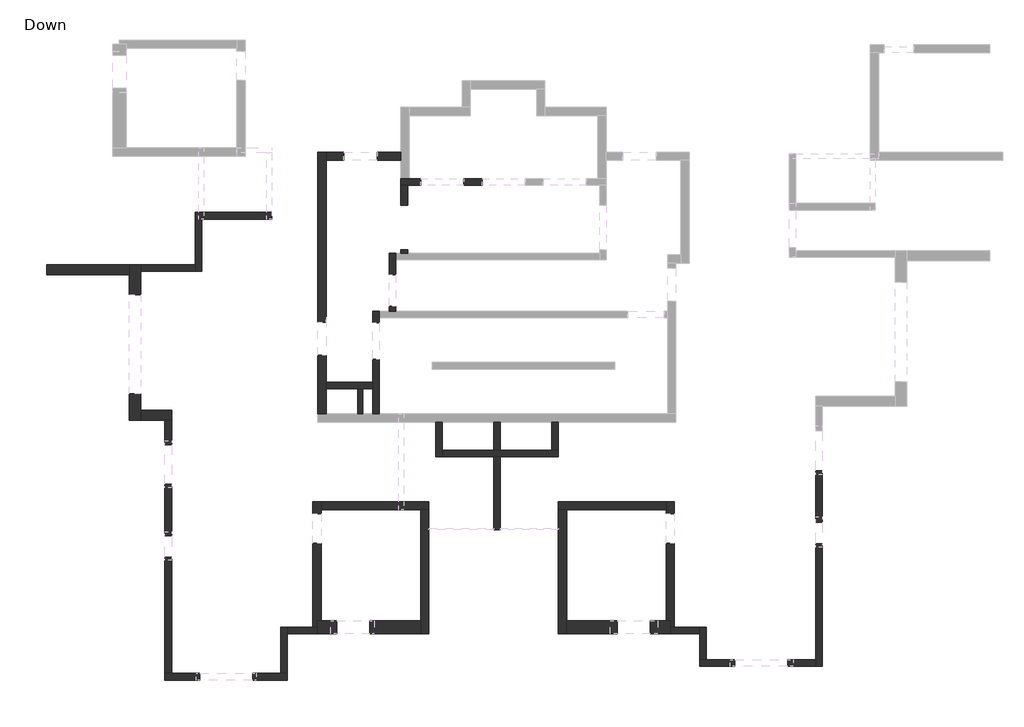
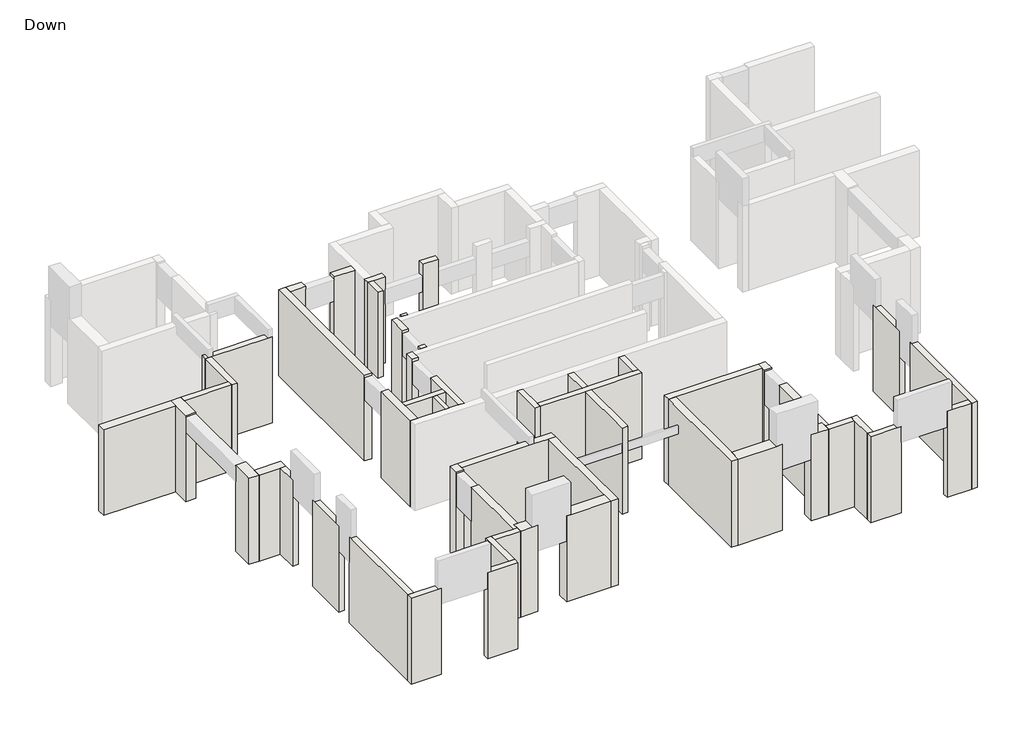
# One storey, part 1 of 3: 51 walls.
"""IFC4 building model written with IfcOpenShell, lengths in millimetres."""

from ifc_helpers import new_model, si_unit, origin, origin_with_axes, place, context, project, spatial, polyline, outline, extrude, faceted_brep, element, save

model = new_model("IFC4")

# Units and contexts
model_context = context("Model", 3, world=origin())
ifc_project = project(units=[si_unit("LENGTHUNIT", "METRE", prefix="MILLI")], contexts=[model_context])

# Site, building, storey
site = spatial("IfcSite", under=ifc_project)
building = spatial("IfcBuilding", under=site)
storey = spatial("IfcBuildingStorey", under=building, Name="Down", Elevation=0.0)

# Walls
placement = place(None, origin())
element("IfcWall", 1, ObjectType="15", at=placement, inside=storey, context=model_context, shape_type="SweptSolid", body=[
    extrude(outline(polyline([(-19501.573099, -7874.1201217), (-19501.573099, -7122.1728784), (-19351.573099, -7122.1728784), (-19351.573099, -7874.1201217), (-19501.573099, -7874.1201217)])), origin_with_axes(), (0.0, 0.0, 1.0), 3150.0),
])
element("IfcWall", 2, ObjectType="20", at=placement, inside=storey, context=model_context, shape_type="Brep", body=[
    faceted_brep([(-22100.9487358, -1784.190313, 0.0), (-24415.0622873, -1784.190313, 0.0), (-24415.0622873, -1784.190313, 3150.0), (-24310.0622873, -1784.190313, 3150.0), (-24160.0622873, -1784.190313, 3150.0), (-22250.9487358, -1784.190313, 3150.0), (-22100.9487358, -1784.190313, 3150.0), (-22100.9487358, -1784.190313, 2850.0), (-22100.9487358, -1984.190313, 0.0), (-22100.9487358, -1984.190313, 2950.0), (-22100.9487358, -1984.190313, 3150.0), (-22250.9487358, -1984.190313, 3150.0), (-24160.0622873, -1984.190313, 3150.0), (-24215.0622873, -1984.190313, 3150.0), (-24310.0622873, -1984.190313, 3150.0), (-24415.0622873, -1984.190313, 3150.0), (-24415.0622873, -1984.190313, 0.0), (-24215.0622873, -1984.190313, 0.0)], [[[0, 1, 2, 3, 4, 5, 6, 7]], [[8, 9, 10, 11, 12, 13, 14, 15, 16, 17]], [[1, 0, 8, 17, 16]], [[6, 5, 4, 3, 2, 15, 14, 13, 12, 11, 10]], [[0, 7, 6, 10, 9, 8]], [[2, 1, 16, 15]]]),
])
element("IfcWall", 3, ObjectType="20", at=placement, inside=storey, context=model_context, shape_type="Brep", body=[
    faceted_brep([(-24415.0622873, -1984.190313, 0.0), (-24415.0622873, -3366.82362, 0.0), (-24415.0622873, -3566.82362, 0.0), (-24415.0622873, -3566.82362, 3150.0), (-24415.0622873, -3366.82362, 3150.0), (-24415.0622873, -1984.190313, 3150.0), (-24215.0622873, -1984.190313, 0.0), (-24215.0622873, -1984.190313, 2950.0), (-24215.0622873, -1984.190313, 3150.0), (-24215.0622873, -3566.82362, 3150.0), (-24215.0622873, -3566.82362, 2950.0), (-24215.0622873, -3566.82362, 0.0)], [[[0, 1, 2, 3, 4, 5]], [[6, 7, 8, 9, 10, 11]], [[2, 1, 0, 6, 11]], [[5, 4, 3, 9, 8]], [[0, 5, 8, 7, 6]], [[3, 2, 11, 10, 9]]]),
])
element("IfcWall", 4, ObjectType="20", at=placement, inside=storey, context=model_context, shape_type="Brep", body=[
    faceted_brep([(-24415.0622873, -3366.82362, 0.0), (-26062.7923903, -3366.82362, 0.0), (-26062.7923903, -3366.82362, 3150.0), (-24415.0622873, -3366.82362, 3150.0), (-24415.0622873, -3566.82362, 0.0), (-24415.0622873, -3566.82362, 3150.0), (-26062.7923903, -3566.82362, 3150.0), (-26062.7923903, -3566.82362, 2950.0), (-26062.7923903, -3566.82362, 0.0)], [[[0, 1, 2, 3]], [[4, 5, 6, 7, 8]], [[1, 0, 4, 8]], [[3, 2, 6, 5]], [[0, 3, 5, 4]], [[2, 1, 8, 7, 6]]]),
])
element("IfcWall", 5, ObjectType="20", at=placement, inside=storey, context=model_context, shape_type="Brep", body=[
    faceted_brep([(-25331.1270445, -12221.0520814, 0.0), (-25331.1270445, -15727.4032645, 0.0), (-25331.1270445, -15727.4032645, 3150.0), (-25331.1270445, -12301.0520814, 3150.0), (-25331.1270445, -12221.0520814, 3150.0), (-25331.1270445, -12221.0520814, 2220.0), (-25131.1270445, -12221.0520814, 0.0), (-25131.1270445, -12221.0520814, 2220.0), (-25131.1270445, -12221.0520814, 3150.0), (-25131.1270445, -12301.0520814, 3150.0), (-25131.1270445, -15727.4032645, 3150.0), (-25131.1270445, -15727.4032645, 2950.0), (-25131.1270445, -15727.4032645, 0.0)], [[[0, 1, 2, 3, 4, 5]], [[6, 7, 8, 9, 10, 11, 12]], [[1, 0, 6, 12]], [[4, 3, 2, 10, 9, 8]], [[0, 5, 4, 8, 7, 6]], [[2, 1, 12, 11, 10]]]),
])
element("IfcWall", 6, ObjectType="20", at=placement, inside=storey, context=model_context, shape_type="Brep", body=[
    faceted_brep([(-22676.7174441, -15927.4032645, 0.0), (-21625.2739934, -15927.4032645, 0.0), (-21625.2739934, -15927.4032645, 3150.0), (-22565.2739934, -15927.4032645, 3150.0), (-22676.7174441, -15927.4032645, 3150.0), (-22676.7174441, -15927.4032645, 2570.0), (-22676.7174441, -15727.4032645, 0.0), (-22676.7174441, -15727.4032645, 2570.0), (-22676.7174441, -15727.4032645, 3150.0), (-22565.2739934, -15727.4032645, 3150.0), (-21825.2739934, -15727.4032645, 3150.0), (-21625.2739934, -15727.4032645, 3150.0), (-21625.2739934, -15727.4032645, 0.0), (-21825.2739934, -15727.4032645, 0.0)], [[[0, 1, 2, 3, 4, 5]], [[6, 7, 8, 9, 10, 11, 12, 13]], [[1, 0, 6, 13, 12]], [[4, 3, 2, 11, 10, 9, 8]], [[0, 5, 4, 8, 7, 6]], [[2, 1, 12, 11]]]),
])
element("IfcWall", 7, ObjectType="20", at=placement, inside=storey, context=model_context, shape_type="Brep", body=[
    faceted_brep([(-21625.2739934, -15727.4032645, 0.0), (-21625.2739934, -14534.8752446, 0.0), (-21625.2739934, -14334.8752446, 0.0), (-21625.2739934, -14334.8752446, 3150.0), (-21625.2739934, -14534.8752446, 3150.0), (-21625.2739934, -15727.4032645, 3150.0), (-21825.2739934, -15727.4032645, 0.0), (-21825.2739934, -15727.4032645, 2950.0), (-21825.2739934, -15727.4032645, 3150.0), (-21825.2739934, -14334.8752446, 3150.0), (-21825.2739934, -14334.8752446, 2950.0), (-21825.2739934, -14334.8752446, 0.0)], [[[0, 1, 2, 3, 4, 5]], [[6, 7, 8, 9, 10, 11]], [[2, 1, 0, 6, 11]], [[5, 4, 3, 9, 8]], [[0, 5, 8, 7, 6]], [[3, 2, 11, 10, 9]]]),
])
element("IfcWall", 8, ObjectType="20", at=placement, inside=storey, context=model_context, shape_type="Brep", body=[
    faceted_brep([(-21625.2739934, -14534.8752446, 0.0), (-20729.0071531, -14534.8752446, 0.0), (-20729.0071531, -14534.8752446, 3150.0), (-21625.2739934, -14534.8752446, 3150.0), (-21625.2739934, -14334.8752446, 0.0), (-21625.2739934, -14334.8752446, 3150.0), (-20854.0071531, -14334.8752446, 3150.0), (-20729.0071531, -14334.8752446, 3150.0), (-20729.0071531, -14334.8752446, 0.0), (-20854.0071531, -14334.8752446, 0.0)], [[[0, 1, 2, 3]], [[4, 5, 6, 7, 8, 9]], [[1, 0, 4, 9, 8]], [[2, 1, 8, 7]], [[3, 2, 7, 6, 5]], [[0, 3, 5, 4]]]),
])
element("IfcWall", 9, ObjectType="20", at=placement, inside=storey, context=model_context, shape_type="Brep", body=[
    faceted_brep([(-5648.4371316, -11806.6175745, 0.0), (-5648.4371316, -15307.4032645, 0.0), (-5648.4371316, -15507.4032645, 0.0), (-5648.4371316, -15507.4032645, 3150.0), (-5648.4371316, -15307.4032645, 3150.0), (-5648.4371316, -11906.6175745, 3150.0), (-5648.4371316, -11806.6175745, 3150.0), (-5648.4371316, -11806.6175745, 2220.0), (-5448.4371316, -11806.6175745, 0.0), (-5448.4371316, -11806.6175745, 2220.0), (-5448.4371316, -11806.6175745, 3150.0), (-5448.4371316, -11906.6175745, 3150.0), (-5448.4371316, -15507.4032645, 3150.0), (-5448.4371316, -15507.4032645, 0.0)], [[[0, 1, 2, 3, 4, 5, 6, 7]], [[8, 9, 10, 11, 12, 13]], [[2, 1, 0, 8, 13]], [[6, 5, 4, 3, 12, 11, 10]], [[0, 7, 6, 10, 9, 8]], [[3, 2, 13, 12]]]),
])
element("IfcWall", 10, ObjectType="20", at=placement, inside=storey, context=model_context, shape_type="Brep", body=[
    faceted_brep([(-8093.7920507, -15307.4032645, 0.0), (-8953.7920507, -15307.4032645, 0.0), (-9153.7920507, -15307.4032645, 0.0), (-9153.7920507, -15307.4032645, 3150.0), (-8953.7920507, -15307.4032645, 3150.0), (-8233.7920507, -15307.4032645, 3150.0), (-8093.7920507, -15307.4032645, 3150.0), (-8093.7920507, -15307.4032645, 2570.0), (-8093.7920507, -15507.4032645, 0.0), (-8093.7920507, -15507.4032645, 2570.0), (-8093.7920507, -15507.4032645, 3150.0), (-8233.7920507, -15507.4032645, 3150.0), (-9153.7920507, -15507.4032645, 3150.0), (-9153.7920507, -15507.4032645, 0.0)], [[[0, 1, 2, 3, 4, 5, 6, 7]], [[8, 9, 10, 11, 12, 13]], [[2, 1, 0, 8, 13]], [[6, 5, 4, 3, 12, 11, 10]], [[0, 7, 6, 10, 9, 8]], [[3, 2, 13, 12]]]),
])
element("IfcWall", 11, ObjectType="20", at=placement, inside=storey, context=model_context, shape_type="Brep", body=[
    faceted_brep([(-8953.7920507, -15307.4032645, 0.0), (-8953.7920507, -14334.8752446, 0.0), (-8953.7920507, -14334.8752446, 2950.0), (-8953.7920507, -14334.8752446, 3150.0), (-8953.7920507, -15307.4032645, 3150.0), (-8953.7920507, -15307.4032645, 2950.0), (-9153.7920507, -15307.4032645, 0.0), (-9153.7920507, -15307.4032645, 3150.0), (-9153.7920507, -14534.8752446, 3150.0), (-9153.7920507, -14334.8752446, 3150.0), (-9153.7920507, -14334.8752446, 0.0), (-9153.7920507, -14534.8752446, 0.0)], [[[0, 1, 2, 3, 4, 5]], [[6, 7, 8, 9, 10, 11]], [[1, 0, 6, 11, 10]], [[4, 3, 9, 8, 7]], [[0, 5, 4, 7, 6]], [[3, 2, 1, 10, 9]]]),
])
element("IfcWall", 12, ObjectType="20", at=placement, inside=storey, context=model_context, shape_type="Brep", body=[
    faceted_brep([(-9153.7920507, -14334.8752446, 0.0), (-9925.0588909, -14334.8752446, 0.0), (-10050.0588909, -14334.8752446, 0.0), (-10050.0588909, -14334.8752446, 3150.0), (-9925.0588909, -14334.8752446, 3150.0), (-9153.7920507, -14334.8752446, 3150.0), (-9153.7920507, -14534.8752446, 0.0), (-9153.7920507, -14534.8752446, 3150.0), (-10050.0588909, -14534.8752446, 3150.0), (-10050.0588909, -14534.8752446, 0.0)], [[[0, 1, 2, 3, 4, 5]], [[6, 7, 8, 9]], [[2, 1, 0, 6, 9]], [[3, 2, 9, 8]], [[5, 4, 3, 8, 7]], [[0, 5, 7, 6]]]),
])
element("IfcWall", 13, ObjectType="20", at=placement, inside=storey, context=model_context, shape_type="Brep", body=[
    faceted_brep([(-19043.2746727, -4768.7708633, 0.0), (-19043.2746727, -5119.2520135, 0.0), (-19043.2746727, -5119.2520135, 2250.0), (-19043.2746727, -5119.2520135, 3050.0), (-19043.2746727, -5119.2520135, 3150.0), (-19043.2746727, -4768.7708633, 3150.0), (-19043.2746727, -4768.7708633, 2950.0), (-18843.2746727, -4768.7708633, 0.0), (-18843.2746727, -4768.7708633, 3150.0), (-18843.2746727, -4968.7708633, 3150.0), (-18843.2746727, -5119.2520135, 3150.0), (-18843.2746727, -5119.2520135, 2950.0), (-18843.2746727, -5119.2520135, 2250.0), (-18843.2746727, -5119.2520135, 0.0), (-18843.2746727, -4968.7708633, 0.0), (-18848.2746727, -5119.2520135, 3150.0)], [[[0, 1, 2, 3, 4, 5, 6]], [[7, 8, 9, 10, 11, 12, 13, 14]], [[1, 0, 7, 14, 13]], [[4, 3, 2, 1, 13, 12, 11, 10, 15]], [[5, 4, 15, 10, 9, 8]], [[0, 6, 5, 8, 7]]]),
])
element("IfcWall", 14, ObjectType="20", at=placement, inside=storey, context=model_context, shape_type="Brep", body=[
    faceted_brep([(-19043.2746727, -6221.210578, 0.0), (-19043.2746727, -6922.1728784, 0.0), (-19043.2746727, -7122.1728784, 0.0), (-19043.2746727, -7874.1201217, 0.0), (-19043.2746727, -7874.1201217, 3150.0), (-19043.2746727, -7122.1728784, 3150.0), (-19043.2746727, -6922.1728784, 3150.0), (-19043.2746727, -6221.210578, 3150.0), (-19043.2746727, -6221.210578, 3050.0), (-19043.2746727, -6221.210578, 2250.0), (-18843.2746727, -6221.210578, 0.0), (-18843.2746727, -6221.210578, 2250.0), (-18843.2746727, -6221.210578, 2950.0), (-18843.2746727, -6221.210578, 3150.0), (-18843.2746727, -7874.1201217, 3150.0), (-18843.2746727, -7874.1201217, 2950.0), (-18843.2746727, -7874.1201217, 0.0), (-18848.2746727, -6221.210578, 3150.0)], [[[0, 1, 2, 3, 4, 5, 6, 7, 8, 9]], [[10, 11, 12, 13, 14, 15, 16]], [[3, 2, 1, 0, 10, 16]], [[7, 6, 5, 4, 14, 13, 17]], [[0, 9, 8, 7, 17, 13, 12, 11, 10]], [[4, 3, 16, 15, 14]]]),
])
element("IfcWall", 15, ObjectType="20", at=placement, inside=storey, context=model_context, shape_type="Brep", body=[
    faceted_brep([(-19043.2746727, -6922.1728784, 0.0), (-20453.0108891, -6922.1728784, 0.0), (-20453.0108891, -6922.1728784, 2950.0), (-20453.0108891, -6922.1728784, 3150.0), (-19043.2746727, -6922.1728784, 3150.0), (-19043.2746727, -6922.1728784, 2950.0), (-19043.2746727, -7122.1728784, 0.0), (-19043.2746727, -7122.1728784, 3150.0), (-19351.573099, -7122.1728784, 3150.0), (-19501.573099, -7122.1728784, 3150.0), (-20453.0108891, -7122.1728784, 3150.0), (-20453.0108891, -7122.1728784, 0.0), (-19501.573099, -7122.1728784, 0.0), (-19351.573099, -7122.1728784, 0.0)], [[[0, 1, 2, 3, 4, 5]], [[6, 7, 8, 9, 10, 11, 12, 13]], [[1, 0, 6, 13, 12, 11]], [[4, 3, 10, 9, 8, 7]], [[3, 2, 1, 11, 10]], [[0, 5, 4, 7, 6]]]),
])
element("IfcWall", 16, ObjectType="20", at=placement, inside=storey, context=model_context, shape_type="Brep", body=[
    faceted_brep([(-15740.0028511, -762.4310014, 0.0), (-16290.9821333, -762.4310014, 0.0), (-16290.9821333, -762.4310014, 2150.0), (-16290.9821333, -762.4310014, 2700.0), (-16290.9821333, -762.4310014, 3150.0), (-15740.0028511, -762.4310014, 3150.0), (-15740.0028511, -762.4310014, 2700.0), (-15740.0028511, -762.4310014, 2150.0), (-15740.0028511, -962.4310014, 0.0), (-15740.0028511, -962.4310014, 2150.0), (-15740.0028511, -962.4310014, 2700.0), (-15740.0028511, -962.4310014, 3150.0), (-16290.9821333, -962.4310014, 3150.0), (-16290.9821333, -962.4310014, 2700.0), (-16290.9821333, -962.4310014, 2150.0), (-16290.9821333, -962.4310014, 0.0)], [[[0, 1, 2, 3, 4, 5, 6, 7]], [[8, 9, 10, 11, 12, 13, 14, 15]], [[1, 0, 8, 15]], [[4, 3, 2, 1, 15, 14, 13, 12]], [[5, 4, 12, 11]], [[0, 7, 6, 5, 11, 10, 9, 8]]]),
])
element("IfcWall", 17, ObjectType="20", at=placement, inside=storey, context=model_context, shape_type="Brep", body=[
    faceted_brep([(-17593.4388298, -762.4310014, 0.0), (-17944.4124515, -762.4310014, 0.0), (-18194.4124515, -762.4310014, 0.0), (-18194.4124515, -762.4310014, 3150.0), (-17944.4124515, -762.4310014, 3150.0), (-17593.4388298, -762.4310014, 3150.0), (-17593.4388298, -762.4310014, 2700.0), (-17593.4388298, -762.4310014, 2150.0), (-17593.4388298, -962.4310014, 0.0), (-17593.4388298, -962.4310014, 2150.0), (-17593.4388298, -962.4310014, 2700.0), (-17593.4388298, -962.4310014, 3150.0), (-17994.4124515, -962.4310014, 3150.0), (-18194.4124515, -962.4310014, 3150.0), (-18194.4124515, -962.4310014, 0.0), (-17994.4124515, -962.4310014, 0.0)], [[[0, 1, 2, 3, 4, 5, 6, 7]], [[8, 9, 10, 11, 12, 13, 14, 15]], [[2, 1, 0, 8, 15, 14]], [[5, 4, 3, 13, 12, 11]], [[0, 7, 6, 5, 11, 10, 9, 8]], [[3, 2, 14, 13]]]),
])
element("IfcWall", 18, ObjectType="20", at=placement, inside=storey, context=model_context, shape_type="Brep", body=[
    faceted_brep([(-18194.4124515, -962.4310014, 0.0), (-18194.4124515, -1563.404623, 0.0), (-18194.4124515, -1563.404623, 2950.0), (-18194.4124515, -1563.404623, 3150.0), (-18194.4124515, -962.4310014, 3150.0), (-17994.4124515, -962.4310014, 0.0), (-17994.4124515, -962.4310014, 3150.0), (-17994.4124515, -1563.404623, 3150.0), (-17994.4124515, -1563.404623, 2950.0), (-17994.4124515, -1563.404623, 0.0)], [[[0, 1, 2, 3, 4]], [[5, 6, 7, 8, 9]], [[1, 0, 5, 9]], [[3, 2, 1, 9, 8, 7]], [[4, 3, 7, 6]], [[0, 4, 6, 5]]]),
])
element("IfcWall", 19, ObjectType="20", at=placement, inside=storey, context=model_context, shape_type="Brep", body=[
    faceted_brep([(-18193.9143195, -2915.3348845, 0.0), (-18193.9143195, -3015.8216954, 0.0), (-18193.9143195, -3015.8216954, 2950.0), (-18193.9143195, -3015.8216954, 3150.0), (-18193.9143195, -2915.3348845, 3150.0), (-18193.9143195, -2915.3348845, 2950.0), (-17993.9143195, -2915.3348845, 0.0), (-17993.9143195, -2915.3348845, 2950.0), (-17993.9143195, -2915.3348845, 3150.0), (-17993.9143195, -3015.8216954, 3150.0), (-17993.9143195, -3015.8216954, 2950.0), (-17993.9143195, -3015.8216954, 0.0)], [[[0, 1, 2, 3, 4, 5]], [[6, 7, 8, 9, 10, 11]], [[1, 0, 6, 11]], [[4, 3, 9, 8]], [[0, 5, 4, 8, 7, 6]], [[3, 2, 1, 11, 10, 9]]]),
])
element("IfcWall", 20, ObjectType="20", at=placement, inside=storey, context=model_context, shape_type="Brep", body=[
    faceted_brep([(-18550.1013454, -3015.8216954, 0.0), (-18550.1013454, -3666.8122988, 0.0), (-18550.1013454, -3666.8122988, 2250.0), (-18550.1013454, -3666.8122988, 3050.0), (-18550.1013454, -3666.8122988, 3150.0), (-18550.1013454, -3015.8216954, 3150.0), (-18550.1013454, -3015.8216954, 2950.0), (-18350.1013454, -3015.8216954, 0.0), (-18350.1013454, -3015.8216954, 3150.0), (-18350.1013454, -3215.8216954, 3150.0), (-18350.1013454, -3666.8122988, 3150.0), (-18350.1013454, -3666.8122988, 3050.0), (-18350.1013454, -3666.8122988, 2250.0), (-18350.1013454, -3666.8122988, 0.0), (-18350.1013454, -3215.8216954, 0.0)], [[[0, 1, 2, 3, 4, 5, 6]], [[7, 8, 9, 10, 11, 12, 13, 14]], [[1, 0, 7, 14, 13]], [[4, 3, 2, 1, 13, 12, 11, 10]], [[5, 4, 10, 9, 8]], [[0, 6, 5, 8, 7]]]),
])
element("IfcWall", 21, ObjectType="20", at=placement, inside=storey, context=model_context, shape_type="Brep", body=[
    faceted_brep([(-17147.6559701, -8124.1201217, 0.0), (-17147.6559701, -9176.0843468, 0.0), (-17147.6559701, -9176.0843468, 3000.0), (-17147.6559701, -9176.0843468, 3150.0), (-17147.6559701, -8124.1201217, 3150.0), (-17147.6559701, -8124.1201217, 3000.0), (-16947.6559701, -8124.1201217, 0.0), (-16947.6559701, -8124.1201217, 3150.0), (-16947.6559701, -8976.0843468, 3150.0), (-16947.6559701, -9176.0843468, 3150.0), (-16947.6559701, -9176.0843468, 0.0), (-16947.6559701, -8976.0843468, 0.0)], [[[0, 1, 2, 3, 4, 5]], [[6, 7, 8, 9, 10, 11]], [[1, 0, 6, 11, 10]], [[4, 3, 9, 8, 7]], [[0, 5, 4, 7, 6]], [[3, 2, 1, 10, 9]]]),
])
element("IfcWall", 22, ObjectType="20", at=placement, inside=storey, context=model_context, shape_type="Brep", body=[
    faceted_brep([(-16947.6559701, -9176.0843468, 0.0), (-15389.5217009, -9176.0843468, 0.0), (-15189.5217009, -9176.0843468, 0.0), (-13431.410074, -9176.0843468, 0.0), (-13431.410074, -9176.0843468, 3000.0), (-13431.410074, -9176.0843468, 3150.0), (-15189.5217009, -9176.0843468, 3150.0), (-15389.5217009, -9176.0843468, 3150.0), (-16947.6559701, -9176.0843468, 3150.0), (-16947.6559701, -8976.0843468, 0.0), (-16947.6559701, -8976.0843468, 3150.0), (-15389.5443432, -8976.0843468, 3150.0), (-15189.5443432, -8976.0843468, 3150.0), (-13631.410074, -8976.0843468, 3150.0), (-13431.410074, -8976.0843468, 3150.0), (-13431.410074, -8976.0843468, 0.0), (-13631.410074, -8976.0843468, 0.0), (-15189.5443432, -8976.0843468, 0.0), (-15389.5443432, -8976.0843468, 0.0)], [[[0, 1, 2, 3, 4, 5, 6, 7, 8]], [[9, 10, 11, 12, 13, 14, 15, 16, 17, 18]], [[3, 2, 1, 0, 9, 18, 17, 16, 15]], [[8, 7, 6, 5, 14, 13, 12, 11, 10]], [[0, 8, 10, 9]], [[5, 4, 3, 15, 14]]]),
])
element("IfcWall", 23, ObjectType="20", at=placement, inside=storey, context=model_context, shape_type="Brep", body=[
    faceted_brep([(-13431.410074, -8976.0843468, 0.0), (-13431.410074, -8124.1201217, 0.0), (-13431.410074, -8124.1201217, 3000.0), (-13431.410074, -8124.1201217, 3150.0), (-13431.410074, -8976.0843468, 3150.0), (-13631.410074, -8976.0843468, 0.0), (-13631.410074, -8976.0843468, 3150.0), (-13631.410074, -8124.1201217, 3150.0), (-13631.410074, -8124.1201217, 0.0)], [[[0, 1, 2, 3, 4]], [[5, 6, 7, 8]], [[1, 0, 5, 8]], [[4, 3, 7, 6]], [[0, 4, 6, 5]], [[3, 2, 1, 8, 7]]]),
])
element("IfcWall", 24, ObjectType="20", at=placement, inside=storey, context=model_context, shape_type="SweptSolid", body=[
    extrude(outline(polyline([(-15389.5443432, -8976.0843468), (-15389.5443432, -8124.1201217), (-15189.5443432, -8124.1201217), (-15189.5443432, -8976.0843468), (-15389.5443432, -8976.0843468)])), origin_with_axes(), (0.0, 0.0, 1.0), 3150.0),
])
element("IfcWall", 25, ObjectType="20", at=placement, inside=storey, context=model_context, shape_type="Brep", body=[
    faceted_brep([(-15389.5217009, -9176.0843468, 0.0), (-15389.5217009, -11388.1261219, 0.0), (-15389.5217009, -11388.1261219, 2250.0), (-15389.5217009, -11388.1261219, 2550.0), (-15389.5217009, -11388.1261219, 3150.0), (-15389.5217009, -11338.1261219, 3150.0), (-15389.5217009, -9176.0843468, 3150.0), (-15389.5217009, -9176.0843468, 3000.0), (-15189.5217009, -9176.0843468, 0.0), (-15189.5217009, -9176.0843468, 3000.0), (-15189.5217009, -9176.0843468, 3150.0), (-15189.5217009, -11338.1261219, 3150.0), (-15189.5217009, -11388.1261219, 3150.0), (-15189.5217009, -11388.1261219, 2550.0), (-15189.5217009, -11388.1261219, 2250.0), (-15189.5217009, -11388.1261219, 0.0)], [[[0, 1, 2, 3, 4, 5, 6, 7]], [[8, 9, 10, 11, 12, 13, 14, 15]], [[1, 0, 8, 15]], [[4, 3, 2, 1, 15, 14, 13, 12]], [[6, 5, 4, 12, 11, 10]], [[0, 7, 6, 10, 9, 8]]]),
])
element("IfcWall", 26, ObjectType="20", at=placement, inside=storey, context=model_context, shape_type="Brep", body=[
    faceted_brep([(-18350.1013454, -4768.7708633, 0.0), (-18350.1013454, -4618.2670707, 0.0), (-18350.1013454, -4618.2670707, 2250.0), (-18350.1013454, -4618.2670707, 3050.0), (-18350.1013454, -4618.2670707, 3150.0), (-18350.1013454, -4768.7708633, 3150.0), (-18350.1013454, -4768.7708633, 2950.0), (-18550.1013454, -4768.7708633, 0.0), (-18550.1013454, -4768.7708633, 2950.0), (-18550.1013454, -4768.7708633, 3150.0), (-18550.1013454, -4618.2670707, 3150.0), (-18550.1013454, -4618.2670707, 3050.0), (-18550.1013454, -4618.2670707, 2250.0), (-18550.1013454, -4618.2670707, 0.0)], [[[0, 1, 2, 3, 4, 5, 6]], [[7, 8, 9, 10, 11, 12, 13]], [[1, 0, 7, 13]], [[4, 3, 2, 1, 13, 12, 11, 10]], [[5, 4, 10, 9]], [[0, 6, 5, 9, 8, 7]]]),
])
element("IfcWall", 27, ObjectType="20", at=placement, inside=storey, context=model_context, shape_type="Brep", body=[
    faceted_brep([(-6499.9032247, -15507.4032645, 0.0), (-5648.4371316, -15507.4032645, 0.0), (-5648.4371316, -15507.4032645, 3150.0), (-6333.7920507, -15507.4032645, 3150.0), (-6499.9032247, -15507.4032645, 3150.0), (-6499.9032247, -15507.4032645, 2570.0), (-6499.9032247, -15307.4032645, 0.0), (-6499.9032247, -15307.4032645, 2570.0), (-6499.9032247, -15307.4032645, 3150.0), (-6333.7920507, -15307.4032645, 3150.0), (-5648.4371316, -15307.4032645, 3150.0), (-5648.4371316, -15307.4032645, 2950.0), (-5648.4371316, -15307.4032645, 0.0)], [[[0, 1, 2, 3, 4, 5]], [[6, 7, 8, 9, 10, 11, 12]], [[1, 0, 6, 12]], [[4, 3, 2, 10, 9, 8]], [[0, 5, 4, 8, 7, 6]], [[2, 1, 12, 11, 10]]]),
])
element("IfcWall", 28, ObjectType="20", at=placement, inside=storey, context=model_context, shape_type="Brep", body=[
    faceted_brep([(-5448.4371316, -11149.2984303, 0.0), (-5448.4371316, -9591.6622931, 0.0), (-5448.4371316, -9591.6622931, 2570.0), (-5448.4371316, -9591.6622931, 3150.0), (-5448.4371316, -9711.6622931, 3150.0), (-5448.4371316, -10986.6175745, 3150.0), (-5448.4371316, -11149.2984303, 3150.0), (-5448.4371316, -11149.2984303, 2220.0), (-5648.4371316, -11149.2984303, 0.0), (-5648.4371316, -11149.2984303, 2220.0), (-5648.4371316, -11149.2984303, 3150.0), (-5648.4371316, -10986.6175745, 3150.0), (-5648.4371316, -9711.6622931, 3150.0), (-5648.4371316, -9591.6622931, 3150.0), (-5648.4371316, -9591.6622931, 2570.0), (-5648.4371316, -9591.6622931, 0.0)], [[[0, 1, 2, 3, 4, 5, 6, 7]], [[8, 9, 10, 11, 12, 13, 14, 15]], [[1, 0, 8, 15]], [[3, 2, 1, 15, 14, 13]], [[6, 5, 4, 3, 13, 12, 11, 10]], [[0, 7, 6, 10, 9, 8]]]),
])
element("IfcWall", 29, ObjectType="20", at=placement, inside=storey, context=model_context, shape_type="Brep", body=[
    faceted_brep([(-25331.6251765, -15927.4032645, 0.0), (-24279.6609514, -15927.4032645, 0.0), (-24279.6609514, -15927.4032645, 2570.0), (-24279.6609514, -15927.4032645, 3150.0), (-24385.2739934, -15927.4032645, 3150.0), (-25331.6251765, -15927.4032645, 3150.0), (-25331.6251765, -15727.4032645, 0.0), (-25331.6251765, -15727.4032645, 3150.0), (-25331.1270445, -15727.4032645, 3150.0), (-25131.1270445, -15727.4032645, 3150.0), (-24385.2739934, -15727.4032645, 3150.0), (-24279.6609514, -15727.4032645, 3150.0), (-24279.6609514, -15727.4032645, 2570.0), (-24279.6609514, -15727.4032645, 0.0), (-25131.1270445, -15727.4032645, 0.0), (-25331.1270445, -15727.4032645, 0.0)], [[[0, 1, 2, 3, 4, 5]], [[6, 7, 8, 9, 10, 11, 12, 13, 14, 15]], [[1, 0, 6, 15, 14, 13]], [[3, 2, 1, 13, 12, 11]], [[5, 4, 3, 11, 10, 9, 8, 7]], [[0, 5, 7, 6]]]),
])
element("IfcWall", 30, ObjectType="20", at=placement, inside=storey, context=model_context, shape_type="Brep", body=[
    faceted_brep([(-25131.1270445, -11570.0841204, 0.0), (-25131.1270445, -10012.4479831, 0.0), (-25131.1270445, -10012.4479831, 2570.0), (-25131.1270445, -10012.4479831, 3150.0), (-25131.1270445, -10112.4479831, 3150.0), (-25131.1270445, -11441.0520814, 3150.0), (-25131.1270445, -11570.0841204, 3150.0), (-25131.1270445, -11570.0841204, 2220.0), (-25331.1270445, -11570.0841204, 0.0), (-25331.1270445, -11570.0841204, 2220.0), (-25331.1270445, -11570.0841204, 3150.0), (-25331.1270445, -11441.0520814, 3150.0), (-25331.1270445, -10112.4479831, 3150.0), (-25331.1270445, -10012.4479831, 3150.0), (-25331.1270445, -10012.4479831, 2570.0), (-25331.1270445, -10012.4479831, 0.0)], [[[0, 1, 2, 3, 4, 5, 6, 7]], [[8, 9, 10, 11, 12, 13, 14, 15]], [[1, 0, 8, 15]], [[3, 2, 1, 15, 14, 13]], [[6, 5, 4, 3, 13, 12, 11, 10]], [[0, 7, 6, 10, 9, 8]]]),
])
element("IfcWall", 31, ObjectType="20", at=placement, inside=storey, context=model_context, shape_type="Brep", body=[
    faceted_brep([(-25131.1270445, -8810.5007399, 0.0), (-25131.1270445, -8064.2310693, 0.0), (-25131.1270445, -8064.2310693, 3150.0), (-25131.1270445, -8692.4479831, 3150.0), (-25131.1270445, -8810.5007399, 3150.0), (-25131.1270445, -8810.5007399, 2570.0), (-25331.1270445, -8810.5007399, 0.0), (-25331.1270445, -8810.5007399, 2570.0), (-25331.1270445, -8810.5007399, 3150.0), (-25331.1270445, -8692.4479831, 3150.0), (-25331.1270445, -8064.2310693, 3150.0), (-25331.1270445, -8064.2310693, 0.0)], [[[0, 1, 2, 3, 4, 5]], [[6, 7, 8, 9, 10, 11]], [[1, 0, 6, 11]], [[4, 3, 2, 10, 9, 8]], [[0, 5, 4, 8, 7, 6]], [[2, 1, 11, 10]]]),
])
element("IfcWall", 32, ObjectType="25", at=placement, inside=storey, context=model_context, shape_type="Brep", body=[
    faceted_brep([(-20604.0071531, -14134.8752446, 0.0), (-20604.0071531, -11794.8752446, 0.0), (-20604.0071531, -11794.8752446, 1900.0), (-20604.0071531, -11794.8752446, 3100.0), (-20604.0071531, -11794.8752446, 3150.0), (-20604.0071531, -14134.8752446, 3150.0), (-20604.0071531, -14134.8752446, 2860.0), (-20854.0071531, -14334.8752446, 0.0), (-20854.0071531, -14334.8752446, 2950.0), (-20854.0071531, -14334.8752446, 3150.0), (-20854.0071531, -11794.8752446, 3150.0), (-20854.0071531, -11794.8752446, 3100.0), (-20854.0071531, -11794.8752446, 1900.0), (-20854.0071531, -11794.8752446, 0.0), (-20729.0071531, -14134.8752446, 0.0), (-20729.0071531, -14334.8752446, 0.0), (-20729.0071531, -14334.8752446, 3150.0), (-20729.0071531, -14134.8752446, 3150.0)], [[[0, 1, 2, 3, 4, 5, 6]], [[7, 8, 9, 10, 11, 12, 13]], [[1, 0, 14, 15, 7, 13]], [[4, 3, 2, 1, 13, 12, 11, 10]], [[5, 4, 10, 9, 16, 17]], [[0, 6, 5, 17, 14]], [[17, 16, 15, 14]], [[16, 9, 8, 7, 15]]]),
])
element("IfcWall", 33, ObjectType="25", at=placement, inside=storey, context=model_context, shape_type="Brep", body=[
    faceted_brep([(-20604.0071531, -10898.8059589, 0.0), (-20604.0071531, -10778.5353827, 0.0), (-20604.0071531, -10528.5353827, 0.0), (-20604.0071531, -10528.5353827, 3150.0), (-20604.0071531, -10778.5353827, 3150.0), (-20604.0071531, -10898.8059589, 3150.0), (-20604.0071531, -10898.8059589, 3100.0), (-20604.0071531, -10898.8059589, 1900.0), (-20854.0071531, -10898.8059589, 0.0), (-20854.0071531, -10898.8059589, 1900.0), (-20854.0071531, -10898.8059589, 3100.0), (-20854.0071531, -10898.8059589, 3150.0), (-20854.0071531, -10528.5353827, 3150.0), (-20854.0071531, -10528.5353827, 2950.0), (-20854.0071531, -10528.5353827, 0.0)], [[[0, 1, 2, 3, 4, 5, 6, 7]], [[8, 9, 10, 11, 12, 13, 14]], [[2, 1, 0, 8, 14]], [[5, 4, 3, 12, 11]], [[0, 7, 6, 5, 11, 10, 9, 8]], [[3, 2, 14, 13, 12]]]),
])
element("IfcWall", 34, ObjectType="25", at=placement, inside=storey, context=model_context, shape_type="Brep", body=[
    faceted_brep([(-20604.0071531, -10778.5353827, 0.0), (-17598.1541021, -10778.5353827, 0.0), (-17348.1541021, -10778.5353827, 0.0), (-17348.1541021, -10778.5353827, 3150.0), (-17598.1541021, -10778.5353827, 3150.0), (-18103.1541021, -10778.5353827, 3150.0), (-18253.1541021, -10778.5353827, 3150.0), (-20604.0071531, -10778.5353827, 3150.0), (-20604.0071531, -10778.5353827, 2860.0), (-20604.0071531, -10528.5353827, 0.0), (-20604.0071531, -10528.5353827, 3150.0), (-18253.1541021, -10528.5353827, 3150.0), (-18103.1541021, -10528.5353827, 3150.0), (-17348.1541021, -10528.5353827, 3150.0), (-17348.1541021, -10528.5353827, 3000.0), (-17348.1541021, -10528.5353827, 0.0)], [[[0, 1, 2, 3, 4, 5, 6, 7, 8]], [[9, 10, 11, 12, 13, 14, 15]], [[2, 1, 0, 9, 15]], [[7, 6, 5, 4, 3, 13, 12, 11, 10]], [[0, 8, 7, 10, 9]], [[3, 2, 15, 14, 13]]]),
])
element("IfcWall", 35, ObjectType="25", at=placement, inside=storey, context=model_context, shape_type="Brep", body=[
    faceted_brep([(-17598.1541021, -10778.5353827, 0.0), (-17598.1541021, -14134.8752446, 0.0), (-17598.1541021, -14534.8752446, 0.0), (-17598.1541021, -14534.8752446, 3150.0), (-17598.1541021, -14134.8752446, 3150.0), (-17598.1541021, -10778.5353827, 3150.0), (-17598.1541021, -10778.5353827, 2860.0), (-17348.1541021, -10778.5353827, 0.0), (-17348.1541021, -10778.5353827, 3150.0), (-17348.1541021, -11338.1261219, 3150.0), (-17348.1541021, -14534.8752446, 3150.0), (-17348.1541021, -14534.8752446, 0.0)], [[[0, 1, 2, 3, 4, 5, 6]], [[7, 8, 9, 10, 11]], [[2, 1, 0, 7, 11]], [[5, 4, 3, 10, 9, 8]], [[0, 6, 5, 8, 7]], [[3, 2, 11, 10]]]),
])
element("IfcWall", 36, ObjectType="25", at=placement, inside=storey, context=model_context, shape_type="Brep", body=[
    faceted_brep([(-9925.0588909, -14334.8752446, 0.0), (-9925.0588909, -11794.8752446, 0.0), (-9925.0588909, -11794.8752446, 1900.0), (-9925.0588909, -11794.8752446, 3100.0), (-9925.0588909, -11794.8752446, 3150.0), (-9925.0588909, -14334.8752446, 3150.0), (-9925.0588909, -14334.8752446, 2950.0), (-10175.0588909, -14134.8526022, 0.0), (-10175.0588909, -14134.8526022, 2860.0), (-10175.0588909, -14134.8526022, 3150.0), (-10175.0588909, -11794.8752446, 3150.0), (-10175.0588909, -11794.8752446, 3100.0), (-10175.0588909, -11794.8752446, 1900.0), (-10175.0588909, -11794.8752446, 0.0), (-10050.0588909, -14334.8752446, 0.0), (-10050.0588909, -14134.8526022, 0.0), (-10050.0588909, -14134.8526022, 3150.0), (-10050.0588909, -14334.8752446, 3150.0)], [[[0, 1, 2, 3, 4, 5, 6]], [[7, 8, 9, 10, 11, 12, 13]], [[1, 0, 14, 15, 7, 13]], [[4, 3, 2, 1, 13, 12, 11, 10]], [[5, 4, 10, 9, 16, 17]], [[0, 6, 5, 17, 14]], [[17, 16, 15, 14]], [[16, 9, 8, 7, 15]]]),
])
element("IfcWall", 37, ObjectType="25", at=placement, inside=storey, context=model_context, shape_type="Brep", body=[
    faceted_brep([(-9925.0588909, -10898.8059589, 0.0), (-9925.0588909, -10528.5353827, 0.0), (-9925.0588909, -10528.5353827, 2950.0), (-9925.0588909, -10528.5353827, 3150.0), (-9925.0588909, -10898.8059589, 3150.0), (-9925.0588909, -10898.8059589, 3100.0), (-9925.0588909, -10898.8059589, 1900.0), (-10175.0588909, -10898.8059589, 0.0), (-10175.0588909, -10898.8059589, 1900.0), (-10175.0588909, -10898.8059589, 3100.0), (-10175.0588909, -10898.8059589, 3150.0), (-10175.0588909, -10778.5353827, 3150.0), (-10175.0588909, -10528.5353827, 3150.0), (-10175.0588909, -10528.5353827, 0.0), (-10175.0588909, -10778.5353827, 0.0)], [[[0, 1, 2, 3, 4, 5, 6]], [[7, 8, 9, 10, 11, 12, 13, 14]], [[1, 0, 7, 14, 13]], [[4, 3, 12, 11, 10]], [[0, 6, 5, 4, 10, 9, 8, 7]], [[3, 2, 1, 13, 12]]]),
])
element("IfcWall", 38, ObjectType="25", at=placement, inside=storey, context=model_context, shape_type="Brep", body=[
    faceted_brep([(-10175.0588909, -10528.5353827, 0.0), (-13430.911942, -10528.5353827, 0.0), (-13430.911942, -10528.5353827, 3000.0), (-13430.911942, -10528.5353827, 3150.0), (-12635.911942, -10528.5353827, 3150.0), (-12485.911942, -10528.5353827, 3150.0), (-10175.0588909, -10528.5353827, 3150.0), (-10175.0588909, -10778.5353827, 0.0), (-10175.0588909, -10778.5353827, 2860.0), (-10175.0588909, -10778.5353827, 3150.0), (-12485.911942, -10778.5353827, 3150.0), (-12635.911942, -10778.5353827, 3150.0), (-13180.911942, -10778.5353827, 3150.0), (-13430.911942, -10778.5353827, 3150.0), (-13430.911942, -10778.5353827, 0.0), (-13180.911942, -10778.5353827, 0.0)], [[[0, 1, 2, 3, 4, 5, 6]], [[7, 8, 9, 10, 11, 12, 13, 14, 15]], [[1, 0, 7, 15, 14]], [[6, 5, 4, 3, 13, 12, 11, 10, 9]], [[0, 6, 9, 8, 7]], [[3, 2, 1, 14, 13]]]),
])
element("IfcWall", 39, ObjectType="25", at=placement, inside=storey, context=model_context, shape_type="Brep", body=[
    faceted_brep([(-13430.911942, -10778.5353827, 0.0), (-13430.911942, -14534.8752446, 0.0), (-13430.911942, -14534.8752446, 3150.0), (-13430.911942, -11338.1261219, 3150.0), (-13430.911942, -10778.5353827, 3150.0), (-13180.911942, -10778.5353827, 0.0), (-13180.911942, -10778.5353827, 2860.0), (-13180.911942, -10778.5353827, 3150.0), (-13180.911942, -14134.8526022, 3150.0), (-13180.911942, -14534.8752446, 3150.0), (-13180.911942, -14534.8752446, 0.0), (-13180.911942, -14134.8752446, 0.0)], [[[0, 1, 2, 3, 4]], [[5, 6, 7, 8, 9, 10, 11]], [[1, 0, 5, 11, 10]], [[4, 3, 2, 9, 8, 7]], [[0, 4, 7, 6, 5]], [[2, 1, 10, 9]]]),
])
element("IfcWall", 40, ObjectType="25", at=placement, inside=storey, context=model_context, shape_type="Brep", body=[
    faceted_brep([(-20703.0108891, -6110.8064118, 0.0), (-20703.0108891, -7874.1201217, 0.0), (-20703.0108891, -7874.1201217, 2950.0), (-20703.0108891, -7874.1201217, 3150.0), (-20703.0108891, -6110.8064118, 3150.0), (-20703.0108891, -6110.8064118, 3050.0), (-20703.0108891, -6110.8064118, 2250.0), (-20453.0108891, -6110.8064118, 0.0), (-20453.0108891, -6110.8064118, 2250.0), (-20453.0108891, -6110.8064118, 2950.0), (-20453.0108891, -6110.8064118, 3150.0), (-20453.0108891, -6922.1728784, 3150.0), (-20453.0108891, -7122.1728784, 3150.0), (-20453.0108891, -7874.1201217, 3150.0), (-20453.0108891, -7874.1201217, 0.0), (-20453.0108891, -7122.1728784, 0.0), (-20453.0108891, -6922.1728784, 0.0), (-20453.5033605, -6110.8064118, 3150.0)], [[[0, 1, 2, 3, 4, 5, 6]], [[7, 8, 9, 10, 11, 12, 13, 14, 15, 16]], [[1, 0, 7, 16, 15, 14]], [[4, 3, 13, 12, 11, 10, 17]], [[0, 6, 5, 4, 17, 10, 9, 8, 7]], [[3, 2, 1, 14, 13]]]),
])
element("IfcWall", 41, ObjectType="25", at=placement, inside=storey, context=model_context, shape_type="Brep", body=[
    faceted_brep([(-20453.5033605, -5109.3573005, 0.0), (-20453.5033605, -210.4611157, 0.0), (-20453.5033605, 39.5388843, 0.0), (-20453.5033605, 39.5388843, 3150.0), (-20453.5033605, -210.4611157, 3150.0), (-20453.5033605, -5109.3573005, 3150.0), (-20453.5033605, -5109.3573005, 3050.0), (-20453.5033605, -5109.3573005, 2950.0), (-20453.5033605, -5109.3573005, 2250.0), (-20703.5033605, -5109.3573005, 0.0), (-20703.5033605, -5109.3573005, 2950.0), (-20703.5033605, -5109.3573005, 3150.0), (-20703.5033605, 39.5388843, 3150.0), (-20703.5033605, 39.5388843, 2950.0), (-20703.5033605, 39.5388843, 0.0), (-20703.0108891, -5109.3573005, 3150.0)], [[[0, 1, 2, 3, 4, 5, 6, 7, 8]], [[9, 10, 11, 12, 13, 14]], [[2, 1, 0, 9, 14]], [[5, 4, 3, 12, 11, 15]], [[0, 8, 7, 6, 5, 15, 11, 10, 9]], [[3, 2, 14, 13, 12]]]),
])
element("IfcWall", 42, ObjectType="25", at=placement, inside=storey, context=model_context, shape_type="Brep", body=[
    faceted_brep([(-20453.5033605, -210.4611157, 0.0), (-19917.1340636, -210.4611157, 0.0), (-19917.1340636, -210.4611157, 2250.0), (-19917.1340636, -210.4611157, 3050.0), (-19917.1340636, -210.4611157, 3150.0), (-20453.5033605, -210.4611157, 3150.0), (-20453.5033605, -210.4611157, 2950.0), (-20453.5033605, 39.5388843, 0.0), (-20453.5033605, 39.5388843, 3150.0), (-19917.1340636, 39.5388843, 3150.0), (-19917.1340636, 39.5388843, 3050.0), (-19917.1340636, 39.5388843, 2250.0), (-19917.1340636, 39.5388843, 0.0)], [[[0, 1, 2, 3, 4, 5, 6]], [[7, 8, 9, 10, 11, 12]], [[1, 0, 7, 12]], [[4, 3, 2, 1, 12, 11, 10, 9]], [[5, 4, 9, 8]], [[0, 6, 5, 8, 7]]]),
])
element("IfcWall", 43, ObjectType="25", at=placement, inside=storey, context=model_context, shape_type="Brep", body=[
    faceted_brep([(-18915.6849523, -210.4611157, 0.0), (-18194.4124515, -210.4611157, 0.0), (-18194.4124515, -210.4611157, 2950.0), (-18194.4124515, -210.4611157, 3150.0), (-18915.6849523, -210.4611157, 3150.0), (-18915.6849523, -210.4611157, 3050.0), (-18915.6849523, -210.4611157, 2250.0), (-18915.6849523, 39.5388843, 0.0), (-18915.6849523, 39.5388843, 2250.0), (-18915.6849523, 39.5388843, 3050.0), (-18915.6849523, 39.5388843, 3150.0), (-18194.4124515, 39.5388843, 3150.0), (-18194.4124515, 39.5388843, 2950.0), (-18194.4124515, 39.5388843, 0.0)], [[[0, 1, 2, 3, 4, 5, 6]], [[7, 8, 9, 10, 11, 12, 13]], [[1, 0, 7, 13]], [[4, 3, 11, 10]], [[0, 6, 5, 4, 10, 9, 8, 7]], [[3, 2, 1, 13, 12, 11]]]),
])
element("IfcWall", 44, ObjectType="30", at=placement, inside=storey, context=model_context, shape_type="Brep", body=[
    faceted_brep([(-26412.7923903, -3366.82362, 0.0), (-28912.7923903, -3366.82362, 0.0), (-28912.7923903, -3366.82362, 3150.0), (-26412.7923903, -3366.82362, 3150.0), (-26412.7923903, -3666.82362, 0.0), (-26412.7923903, -3666.82362, 2770.0), (-26412.7923903, -3666.82362, 3000.0), (-26412.7923903, -3666.82362, 3150.0), (-28912.7923903, -3666.82362, 3150.0), (-28912.7923903, -3666.82362, 0.0)], [[[0, 1, 2, 3]], [[4, 5, 6, 7, 8, 9]], [[1, 0, 4, 9]], [[2, 1, 9, 8]], [[3, 2, 8, 7]], [[0, 3, 7, 6, 5, 4]]]),
])
element("IfcWall", 45, ObjectType="30", at=placement, inside=storey, context=model_context, shape_type="Brep", body=[
    faceted_brep([(-26062.7923903, -8064.2310693, 0.0), (-25331.1270445, -8064.2310693, 0.0), (-25131.1270445, -8064.2310693, 0.0), (-25131.1270445, -8064.2310693, 3150.0), (-25331.1270445, -8064.2310693, 3150.0), (-26062.7923903, -8064.2310693, 3150.0), (-26062.7923903, -7764.2310693, 0.0), (-26062.7923903, -7764.2310693, 2950.0), (-26062.7923903, -7764.2310693, 3150.0), (-25131.1270445, -7764.2310693, 3150.0), (-25131.1270445, -7764.2310693, 2950.0), (-25131.1270445, -7764.2310693, 0.0)], [[[0, 1, 2, 3, 4, 5]], [[6, 7, 8, 9, 10, 11]], [[2, 1, 0, 6, 11]], [[5, 4, 3, 9, 8]], [[0, 5, 8, 7, 6]], [[3, 2, 11, 10, 9]]]),
])
element("IfcWall", 46, ObjectType="35", at=placement, inside=storey, context=model_context, shape_type="Brep", body=[
    faceted_brep([(-26412.7923903, -3366.82362, 0.0), (-26412.7923903, -3666.82362, 0.0), (-26412.7923903, -4267.7859204, 0.0), (-26412.7923903, -4267.7859204, 2550.0), (-26412.7923903, -4267.7859204, 3100.0), (-26412.7923903, -4267.7859204, 3150.0), (-26412.7923903, -3666.82362, 3150.0), (-26412.7923903, -3366.82362, 3150.0), (-26062.7923903, -3366.82362, 0.0), (-26062.7923903, -3366.82362, 3150.0), (-26062.7923903, -3566.82362, 3150.0), (-26062.7923903, -4267.7859204, 3150.0), (-26062.7923903, -4267.7859204, 3100.0), (-26062.7923903, -4267.7859204, 2550.0), (-26062.7923903, -4267.7859204, 0.0), (-26062.7923903, -3566.82362, 0.0)], [[[0, 1, 2, 3, 4, 5, 6, 7]], [[8, 9, 10, 11, 12, 13, 14, 15]], [[2, 1, 0, 8, 15, 14]], [[5, 4, 3, 2, 14, 13, 12, 11]], [[7, 6, 5, 11, 10, 9]], [[0, 7, 9, 8]]]),
])
element("IfcWall", 47, ObjectType="35", at=placement, inside=storey, context=model_context, shape_type="Brep", body=[
    faceted_brep([(-26412.7923903, -7272.6540287, 0.0), (-26412.7923903, -8064.2310693, 0.0), (-26412.7923903, -8064.2310693, 2770.0), (-26412.7923903, -8064.2310693, 3000.0), (-26412.7923903, -8064.2310693, 3150.0), (-26412.7923903, -7272.6540287, 3150.0), (-26412.7923903, -7272.6540287, 3100.0), (-26412.7923903, -7272.6540287, 2550.0), (-26062.7923903, -7272.6540287, 0.0), (-26062.7923903, -7272.6540287, 2550.0), (-26062.7923903, -7272.6540287, 3100.0), (-26062.7923903, -7272.6540287, 3150.0), (-26062.7923903, -7764.2310693, 3150.0), (-26062.7923903, -8064.2310693, 3150.0), (-26062.7923903, -8064.2310693, 0.0), (-26062.7923903, -7764.2310693, 0.0)], [[[0, 1, 2, 3, 4, 5, 6, 7]], [[8, 9, 10, 11, 12, 13, 14, 15]], [[1, 0, 8, 15, 14]], [[5, 4, 13, 12, 11]], [[0, 7, 6, 5, 11, 10, 9, 8]], [[4, 3, 2, 1, 14, 13]]]),
])
element("IfcWall", 48, ObjectType="40", at=placement, inside=storey, context=model_context, shape_type="Brep", body=[
    faceted_brep([(-19133.1541021, -14534.8752446, 0.0), (-17598.1541021, -14534.8752446, 0.0), (-17598.1541021, -14534.8752446, 3150.0), (-18998.1541021, -14534.8752446, 3150.0), (-19133.1541021, -14534.8752446, 3150.0), (-19133.1541021, -14534.8752446, 2230.0), (-19133.1541021, -14134.8752446, 0.0), (-19133.1541021, -14134.8752446, 2230.0), (-19133.1541021, -14134.8752446, 3150.0), (-18998.1541021, -14134.8752446, 3150.0), (-17598.1541021, -14134.8752446, 3150.0), (-17598.1541021, -14134.8752446, 2860.0), (-17598.1541021, -14134.8752446, 0.0)], [[[0, 1, 2, 3, 4, 5]], [[6, 7, 8, 9, 10, 11, 12]], [[1, 0, 6, 12]], [[4, 3, 2, 10, 9, 8]], [[0, 5, 4, 8, 7, 6]], [[2, 1, 12, 11, 10]]]),
])
element("IfcWall", 49, ObjectType="40", at=placement, inside=storey, context=model_context, shape_type="Brep", body=[
    faceted_brep([(-11647.4710574, -14134.8752446, 0.0), (-13180.911942, -14134.8752446, 0.0), (-13180.911942, -14134.8752446, 3150.0), (-11867.4710574, -14134.8752446, 3150.0), (-11647.4710574, -14134.8752446, 3150.0), (-11647.4710574, -14134.8752446, 2230.0), (-11647.4710574, -14534.8752446, 0.0), (-11647.4710574, -14534.8752446, 2230.0), (-11647.4710574, -14534.8752446, 3150.0), (-11867.4710574, -14534.8752446, 3150.0), (-13180.911942, -14534.8752446, 3150.0), (-13180.911942, -14534.8752446, 0.0)], [[[0, 1, 2, 3, 4, 5]], [[6, 7, 8, 9, 10, 11]], [[1, 0, 6, 11]], [[4, 3, 2, 10, 9, 8]], [[0, 5, 4, 8, 7, 6]], [[2, 1, 11, 10]]]),
])
element("IfcWall", 50, ObjectType="40", at=placement, inside=storey, context=model_context, shape_type="Brep", body=[
    faceted_brep([(-10646.8295238, -14534.8526022, 0.0), (-10050.0588909, -14534.8526022, 0.0), (-10050.0588909, -14534.8526022, 3150.0), (-10646.8295238, -14534.8526022, 3150.0), (-10646.8295238, -14134.8526022, 0.0), (-10646.8295238, -14134.8526022, 3150.0), (-10175.0588909, -14134.8526022, 3150.0), (-10050.0588909, -14134.8526022, 3150.0), (-10050.0588909, -14134.8526022, 0.0), (-10175.0588909, -14134.8526022, 0.0), (-10050.0588909, -14334.8752446, 0.0), (-10050.0588909, -14334.8752446, 3150.0)], [[[0, 1, 2, 3]], [[4, 5, 6, 7, 8, 9]], [[1, 0, 4, 9, 8, 10]], [[2, 1, 10, 8, 7, 11]], [[3, 2, 11, 7, 6, 5]], [[0, 3, 5, 4]]]),
])
element("IfcWall", 51, ObjectType="40", at=placement, inside=storey, context=model_context, shape_type="Brep", body=[
    faceted_brep([(-20729.0071531, -14534.8752446, 0.0), (-20132.7346523, -14534.8752446, 0.0), (-20132.7346523, -14534.8752446, 2230.0), (-20132.7346523, -14534.8752446, 3150.0), (-20318.1541021, -14534.8752446, 3150.0), (-20729.0071531, -14534.8752446, 3150.0), (-20729.0071531, -14134.8752446, 0.0), (-20729.0071531, -14134.8752446, 3150.0), (-20604.0071531, -14134.8752446, 3150.0), (-20318.1541021, -14134.8752446, 3150.0), (-20132.7346523, -14134.8752446, 3150.0), (-20132.7346523, -14134.8752446, 2230.0), (-20132.7346523, -14134.8752446, 0.0), (-20604.0071531, -14134.8752446, 0.0), (-20729.0071531, -14334.8752446, 0.0), (-20729.0071531, -14334.8752446, 3150.0)], [[[0, 1, 2, 3, 4, 5]], [[6, 7, 8, 9, 10, 11, 12, 13]], [[1, 0, 14, 6, 13, 12]], [[3, 2, 1, 12, 11, 10]], [[5, 4, 3, 10, 9, 8, 7, 15]], [[0, 5, 15, 7, 6, 14]]]),
])

save(model, "model.ifc")

# Revit data of these elements
# Project information
#   Project Issue Date = "Issue Date"
#   Project Status = "Project Status"
#   Client Name = "לקוח"
#   Project Address = "Enter address here"
#   Project Name = "Project 022"
#   Project Number = "מספר פרויקט"
# Type "15"
#   Layers, outside or top first: 15 cm "Concrete" (function 1)
# Type "20"
#   Layers, outside or top first: 20 cm "Concrete" (function 1)
# Type "25"
#   Layers, outside or top first: 25 cm "Concrete" (function 1)
# Type "30"
#   Layers, outside or top first: 30 cm "Concrete" (function 1)
# Type "35"
#   Layers, outside or top first: 35 cm "Concrete" (function 1)
# Type "40"
#   Layers, outside or top first: 40 cm "Concrete" (function 1)
# Element 1 (IfcWall, "15")
#   Comments = ""
#   Mark = "W124"
#   SOFiSTiK_EdgeZones = "W124"
#   SOFiSTiK_AMG_Comments = ""
#   Top Offset = 0 cm
#   Base Offset = 0 cm
#   wall height = 315 cm
#   SOFiSTiK_AMG_Scheduled = yes
#   SOFiSTiK_AMG_Adjusted = yes
#   Phase Created = New Construction
#   Base Constraint = Down
#   Top Constraint = Typical Floor
#   Materials on its faces: "Concrete"
# Element 2 (IfcWall, "20")
#   Comments = ""
#   Mark = "W24"
#   SOFiSTiK_EdgeZones = "W24"
#   SOFiSTiK_AMG_Comments = ""
#   Top Offset = 0 cm
#   Base Offset = 0 cm
#   wall height = 315 cm
#   SOFiSTiK_AMG_Scheduled = yes
#   SOFiSTiK_AMG_Adjusted = yes
#   Phase Created = New Construction
#   Base Constraint = Down
#   Top Constraint = Typical Floor
#   Materials on its faces: "Concrete"
# Element 3 (IfcWall, "20")
#   Comments = ""
#   Mark = "W25"
#   SOFiSTiK_EdgeZones = "W25"
#   SOFiSTiK_AMG_Comments = ""
#   Top Offset = 0 cm
#   Base Offset = 0 cm
#   wall height = 315 cm
#   SOFiSTiK_AMG_Scheduled = yes
#   SOFiSTiK_AMG_Adjusted = yes
#   Phase Created = New Construction
#   Base Constraint = Down
#   Top Constraint = Typical Floor
#   Materials on its faces: "Concrete"
# Element 4 (IfcWall, "20")
#   Comments = ""
#   Mark = "W26"
#   SOFiSTiK_EdgeZones = "W26"
#   SOFiSTiK_AMG_Comments = ""
#   Top Offset = 0 cm
#   Base Offset = 0 cm
#   wall height = 315 cm
#   SOFiSTiK_AMG_Scheduled = yes
#   SOFiSTiK_AMG_Adjusted = yes
#   Phase Created = New Construction
#   Base Constraint = Down
#   Top Constraint = Typical Floor
#   Materials on its faces: "Concrete"
# Element 5 (IfcWall, "20")
#   Comments = ""
#   Mark = "W27"
#   SOFiSTiK_EdgeZones = "W27"
#   SOFiSTiK_AMG_Comments = ""
#   Top Offset = 0 cm
#   Base Offset = 0 cm
#   wall height = 315 cm
#   SOFiSTiK_AMG_Scheduled = yes
#   SOFiSTiK_AMG_Adjusted = yes
#   Phase Created = New Construction
#   Base Constraint = Down
#   Top Constraint = Typical Floor
#   Materials on its faces: "Concrete"
# Element 6 (IfcWall, "20")
#   Comments = ""
#   Mark = "W28"
#   SOFiSTiK_EdgeZones = "W28"
#   SOFiSTiK_AMG_Comments = ""
#   Top Offset = 0 cm
#   Base Offset = 0 cm
#   wall height = 315 cm
#   SOFiSTiK_AMG_Scheduled = yes
#   SOFiSTiK_AMG_Adjusted = yes
#   Phase Created = New Construction
#   Base Constraint = Down
#   Top Constraint = Typical Floor
#   Materials on its faces: "Concrete"
# Element 7 (IfcWall, "20")
#   Comments = ""
#   Mark = "W29"
#   SOFiSTiK_EdgeZones = "W29"
#   SOFiSTiK_AMG_Comments = ""
#   Top Offset = 0 cm
#   Base Offset = 0 cm
#   wall height = 315 cm
#   SOFiSTiK_AMG_Scheduled = yes
#   SOFiSTiK_AMG_Adjusted = yes
#   Phase Created = New Construction
#   Base Constraint = Down
#   Top Constraint = Typical Floor
#   Materials on its faces: "Concrete"
# Element 8 (IfcWall, "20")
#   Comments = ""
#   Mark = "W30"
#   SOFiSTiK_EdgeZones = "W30"
#   SOFiSTiK_AMG_Comments = ""
#   Top Offset = 0 cm
#   Base Offset = 0 cm
#   wall height = 315 cm
#   SOFiSTiK_AMG_Scheduled = yes
#   SOFiSTiK_AMG_Adjusted = yes
#   Phase Created = New Construction
#   Base Constraint = Down
#   Top Constraint = Typical Floor
#   Materials on its faces: "Concrete"
# Element 9 (IfcWall, "20")
#   Comments = ""
#   Mark = "W31"
#   SOFiSTiK_EdgeZones = "W31"
#   SOFiSTiK_AMG_Comments = ""
#   Top Offset = 0 cm
#   Base Offset = 0 cm
#   wall height = 315 cm
#   SOFiSTiK_AMG_Scheduled = yes
#   SOFiSTiK_AMG_Adjusted = yes
#   Phase Created = New Construction
#   Base Constraint = Down
#   Top Constraint = Typical Floor
#   Materials on its faces: "Concrete"
# Element 10 (IfcWall, "20")
#   Comments = ""
#   Mark = "W32"
#   SOFiSTiK_EdgeZones = "W32"
#   SOFiSTiK_AMG_Comments = ""
#   Top Offset = 0 cm
#   Base Offset = 0 cm
#   wall height = 315 cm
#   SOFiSTiK_AMG_Scheduled = yes
#   SOFiSTiK_AMG_Adjusted = yes
#   Phase Created = New Construction
#   Base Constraint = Down
#   Top Constraint = Typical Floor
#   Materials on its faces: "Concrete"
# Element 11 (IfcWall, "20")
#   Comments = ""
#   Mark = "W33"
#   SOFiSTiK_EdgeZones = "W33"
#   SOFiSTiK_AMG_Comments = ""
#   Top Offset = 0 cm
#   Base Offset = 0 cm
#   wall height = 315 cm
#   SOFiSTiK_AMG_Scheduled = yes
#   SOFiSTiK_AMG_Adjusted = yes
#   Phase Created = New Construction
#   Base Constraint = Down
#   Top Constraint = Typical Floor
#   Materials on its faces: "Concrete"
# Element 12 (IfcWall, "20")
#   Comments = ""
#   Mark = "W34"
#   SOFiSTiK_EdgeZones = "W34"
#   SOFiSTiK_AMG_Comments = ""
#   Top Offset = 0 cm
#   Base Offset = 0 cm
#   wall height = 315 cm
#   SOFiSTiK_AMG_Scheduled = yes
#   SOFiSTiK_AMG_Adjusted = yes
#   Phase Created = New Construction
#   Base Constraint = Down
#   Top Constraint = Typical Floor
#   Materials on its faces: "Concrete"
# Element 13 (IfcWall, "20")
#   Comments = ""
#   Mark = "W42"
#   SOFiSTiK_EdgeZones = "W42"
#   SOFiSTiK_AMG_Comments = ""
#   Top Offset = 0 cm
#   Base Offset = 0 cm
#   wall height = 315 cm
#   SOFiSTiK_AMG_Scheduled = yes
#   SOFiSTiK_AMG_Adjusted = yes
#   Phase Created = New Construction
#   Base Constraint = Down
#   Top Constraint = Typical Floor
#   Materials on its faces: "Concrete"
# Element 14 (IfcWall, "20")
#   Comments = ""
#   Mark = "W43"
#   SOFiSTiK_EdgeZones = "W43"
#   SOFiSTiK_AMG_Comments = ""
#   Top Offset = 0 cm
#   Base Offset = 0 cm
#   wall height = 315 cm
#   SOFiSTiK_AMG_Scheduled = yes
#   SOFiSTiK_AMG_Adjusted = yes
#   Phase Created = New Construction
#   Base Constraint = Down
#   Top Constraint = Typical Floor
#   Materials on its faces: "Concrete"
# Element 15 (IfcWall, "20")
#   Comments = ""
#   Mark = "W44"
#   SOFiSTiK_EdgeZones = "W44"
#   SOFiSTiK_AMG_Comments = ""
#   Top Offset = 0 cm
#   Base Offset = 0 cm
#   wall height = 315 cm
#   SOFiSTiK_AMG_Scheduled = yes
#   SOFiSTiK_AMG_Adjusted = yes
#   Phase Created = New Construction
#   Base Constraint = Down
#   Top Constraint = Typical Floor
#   Materials on its faces: "Concrete"
# Element 16 (IfcWall, "20")
#   Comments = ""
#   Mark = "W47"
#   SOFiSTiK_EdgeZones = "W47"
#   SOFiSTiK_AMG_Comments = ""
#   Top Offset = 0 cm
#   Base Offset = 0 cm
#   wall height = 315 cm
#   SOFiSTiK_AMG_Scheduled = yes
#   SOFiSTiK_AMG_Adjusted = yes
#   Phase Created = New Construction
#   Base Constraint = Down
#   Top Constraint = Typical Floor
#   Materials on its faces: "Concrete"
# Element 17 (IfcWall, "20")
#   Comments = ""
#   Mark = "W48"
#   SOFiSTiK_EdgeZones = "W48"
#   SOFiSTiK_AMG_Comments = ""
#   Top Offset = 0 cm
#   Base Offset = 0 cm
#   wall height = 315 cm
#   SOFiSTiK_AMG_Scheduled = yes
#   SOFiSTiK_AMG_Adjusted = yes
#   Phase Created = New Construction
#   Base Constraint = Down
#   Top Constraint = Typical Floor
#   Materials on its faces: "Concrete"
# Element 18 (IfcWall, "20")
#   Comments = ""
#   Mark = "W49"
#   SOFiSTiK_EdgeZones = "W49"
#   SOFiSTiK_AMG_Comments = ""
#   Top Offset = 0 cm
#   Base Offset = 0 cm
#   wall height = 315 cm
#   SOFiSTiK_AMG_Scheduled = yes
#   SOFiSTiK_AMG_Adjusted = yes
#   Phase Created = New Construction
#   Base Constraint = Down
#   Top Constraint = Typical Floor
#   Materials on its faces: "Concrete"
# Element 19 (IfcWall, "20")
#   Comments = ""
#   Mark = "W53"
#   SOFiSTiK_EdgeZones = "W53"
#   SOFiSTiK_AMG_Comments = "Too Short /"
#   Top Offset = 0 cm
#   Base Offset = 0 cm
#   wall height = 315 cm
#   SOFiSTiK_AMG_Scheduled = yes
#   SOFiSTiK_AMG_Adjusted = yes
#   Phase Created = New Construction
